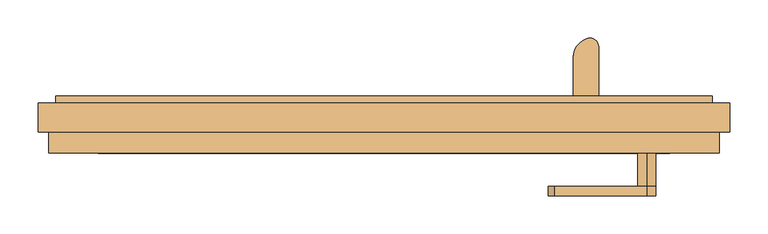
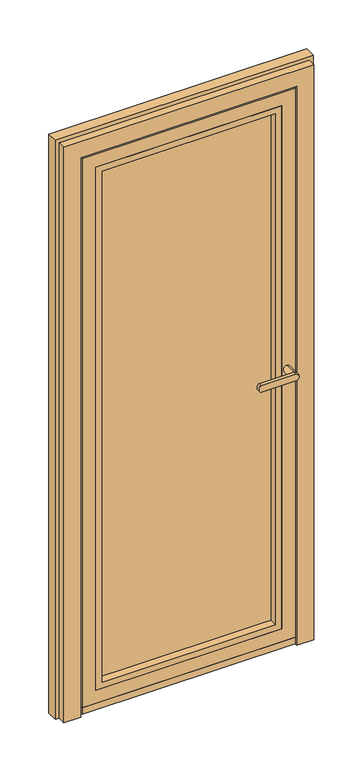
"""IFC4 building model written with IfcOpenShell, lengths in millimetres: door geometry, Schueco_FWS_ADS-75-HD-HI_out_Family-01 : FWS SI insert unit."""

from ifc_helpers import new_model, si_unit, point, frame, frame_2d, origin, place, context, project, spatial, polyline, circle_curve, ellipse_curve, trimmed, segment, composite_curve, outline, extrude, faceted_brep, source, transform, mapped, element, save
from ifc_brep_helpers import plane_surface, cylinder_surface, extruded_surface, advanced_brep


def door_b175160b(model_context):
    return source(origin(), model_context, "Body", "SolidModel", [
        extrude(outline(composite_curve([segment(polyline([(248.3337564, 8.9997177), (248.3337564, 59.1618682)]), True, "CONTINUOUS"), segment(trimmed(circle_curve(frame_2d((275.512174, 59.1618682)), 27.1784177), [point((248.3337564, 59.1618682))], [point((265.9750784, 84.6120194))], False, "CARTESIAN"), True, "CONTINUOUS"), segment(trimmed(circle_curve(frame_2d((270.0525794, 73.7310321)), 11.6198924), [point((265.9750784, 84.6120194))], [point((281.6724718, 73.7310321))], False, "CARTESIAN"), True, "CONTINUOUS"), segment(polyline([(281.6724718, 73.7310321), (281.6724718, 8.9997177), (248.3337564, 8.9997177)]), True, "CONTINUOUS")], self_intersect=False)), frame((0.0, 0.0, 2053.9218203), z_axis=(0.0, 0.0, 1.0), x_axis=(1.0, 0.0, 0.0)), (0.0, 0.0, 1.0), 4.0),
        extrude(outline(polyline([(248.3337564, 12.9997177), (281.6724718, 12.9997177), (281.6724718, 8.9997177), (248.3337564, 8.9997177), (248.3337564, 12.9997177)])), frame((0.0, 0.0, 2023.9218203), z_axis=(0.0, 0.0, 1.0), x_axis=(1.0, 0.0, 0.0)), (0.0, 0.0, 1.0), 30.0),
        extrude(outline(polyline([(248.3337564, 12.9997177), (281.6724718, 12.9997177), (281.6724718, 8.9997177), (248.3337564, 8.9997177), (248.3337564, 12.9997177)])), frame((0.0, 0.0, 49.9218203), z_axis=(0.0, 0.0, 1.0), x_axis=(1.0, 0.0, 0.0)), (0.0, 0.0, 1.0), 30.0),
        extrude(outline(composite_curve([segment(polyline([(248.3337564, 8.9997177), (248.3337564, 59.1618682)]), True, "CONTINUOUS"), segment(trimmed(circle_curve(frame_2d((275.512174, 59.1618682)), 27.1784177), [point((248.3337564, 59.1618682))], [point((265.9750784, 84.6120194))], False, "CARTESIAN"), True, "CONTINUOUS"), segment(trimmed(circle_curve(frame_2d((270.0525794, 73.7310321)), 11.6198924), [point((265.9750784, 84.6120194))], [point((281.6724718, 73.7310321))], False, "CARTESIAN"), True, "CONTINUOUS"), segment(polyline([(281.6724718, 73.7310321), (281.6724718, 8.9997177), (248.3337564, 8.9997177)]), True, "CONTINUOUS")], self_intersect=False)), frame((0.0, 0.0, 45.9218203), z_axis=(0.0, 0.0, 1.0), x_axis=(1.0, 0.0, 0.0)), (0.0, 0.0, 1.0), 4.0),
        advanced_brep(
        [(277.718156, 57.5977179, 2053.9218203), (252.2840039, 72.2821425, 2053.9218203), (277.718156, 57.5977179, 49.9218203), (252.2840039, 72.2821425, 49.9218203)],
        [
            (0, 1, ellipse_curve(frame((265.0010799, 64.9399302, 2053.9218203), z_axis=(0.0, 0.0, 1.0000000000000002), x_axis=(0.5000002582658958, 0.866025254674503, 0.0)), 21.5840887, 14.6844171)),
            (1, 0, ellipse_curve(frame((265.0010799, 64.9399302, 2053.9218203), z_axis=(0.0, 0.0, 1.0000000000000002), x_axis=(0.5000002582658958, 0.866025254674503, 0.0)), 21.5840887, 14.6844171)),
            (2, 3, ellipse_curve(frame((265.0010799, 64.9399302, 49.9218203), z_axis=(0.0, 0.0, -1.0000000000000002), x_axis=(-0.866025254674503, 0.5000002582658958, 0.0)), 14.6844171, 21.5840887)),
            (3, 2, ellipse_curve(frame((265.0010799, 64.9399302, 49.9218203), z_axis=(0.0, 0.0, -1.0000000000000002), x_axis=(-0.866025254674503, 0.5000002582658958, 0.0)), 14.6844171, 21.5840887)),
            (0, 2),
            (3, 1),
        ],
        [
            plane_surface(frame((252.2840039, 72.2821425, 2053.9218203), z_axis=(0.0, 0.0, 1.0000000000000002), x_axis=(0.5000002582658958, 0.866025254674503, 0.0))),
            plane_surface(frame((252.2840039, 72.2821425, 49.9218203), z_axis=(0.0, 0.0, -1.0000000000000002), x_axis=(-0.5000002582658958, -0.866025254674503, 0.0))),
            extruded_surface(trimmed(ellipse_curve(frame((265.0010799, 64.9399302, 49.9218203), z_axis=(0.0, 0.0, -1.0000000000000002), x_axis=(-0.866025254674503, 0.5000002582658958, 0.0)), 14.6844171, 21.5840887), [point((252.2840039, 72.2821425, 49.9218203))], [point((277.718156, 57.5977179, 49.9218203))], True, "CARTESIAN"), (0.0, 0.0, -2004.0), 2004.0),
            extruded_surface(trimmed(ellipse_curve(frame((265.0010799, 64.9399302, 49.9218203), z_axis=(0.0, 0.0, -1.0000000000000002), x_axis=(-0.866025254674503, 0.5000002582658958, 0.0)), 14.6844171, 21.5840887), [point((277.718156, 57.5977179, 49.9218203))], [point((252.2840039, 72.2821425, 49.9218203))], True, "CARTESIAN"), (0.0, 0.0, -2004.0), 2004.0),
        ],
        [
            (0, [[1, 2]]),
            (1, [[3, 4]]),
            (2, [[5, -4, 6, -1]]),
            (3, [[-6, -3, -5, -2]]),
        ],
    ),
        advanced_brep(
        [(345.0010799, -122.0002518, 1030.9991882), (345.0010799, -122.0002518, 1054.9764498), (223.3392873, -122.0002518, 1054.9764498), (223.3392873, -122.0002518, 1030.9991882), (345.0010799, -109.5001648, 1054.9764498), (345.0010799, -109.5001648, 1030.9991882), (223.3392873, -109.5001648, 1030.9991882), (223.3392873, -109.5001648, 1054.9764498), (345.0010799, -66.0002823, 1030.9991882), (345.0010799, -66.0002823, 1054.9764498)],
        [
            (0, 1, circle_curve(frame((345.0010799, -122.0002518, 1042.987819), z_axis=(0.0, -1.0, 0.0), x_axis=(0.0, 0.0, 1.0)), 11.9886308)),
            (1, 2),
            (2, 3, ellipse_curve(frame((223.3392873, -122.0002518, 1042.987819), z_axis=(0.0, -1.0, 0.0), x_axis=(0.0, 0.0, -1.0)), 11.9886308, 7.9050795)),
            (3, 0),
            (4, 5, circle_curve(frame((345.0010799, -109.5001648, 1042.987819), z_axis=(0.0, -1.0, 0.0), x_axis=(0.0, 0.0, 1.0)), 11.9886308)),
            (5, 6),
            (6, 7, ellipse_curve(frame((223.3392873, -109.5001648, 1042.987819), z_axis=(0.0, 1.0, 0.0), x_axis=(0.0, 0.0, -1.0)), 11.9886308, 7.9050795)),
            (7, 4),
            (3, 6),
            (5, 0),
            (2, 7),
            (1, 4),
            (5, 4, circle_curve(frame((345.0010799, -109.5001648, 1042.987819), z_axis=(0.0, -1.0, 0.0), x_axis=(0.0, 0.0, 1.0)), 11.9886308)),
            (8, 9, circle_curve(frame((345.0010799, -66.0002823, 1042.987819), z_axis=(0.0, 1.0, 0.0), x_axis=(0.0, 0.0, 1.0)), 11.9886308)),
            (9, 8, circle_curve(frame((345.0010799, -66.0002823, 1042.987819), z_axis=(0.0, 1.0, 0.0), x_axis=(0.0, 0.0, 1.0)), 11.9886308)),
            (8, 5),
            (4, 9),
        ],
        [
            plane_surface(frame((223.3392873, -122.0002518, 1030.9991882), z_axis=(0.0, -1.0, 0.0), x_axis=(-1.0, 0.0, 0.0))),
            plane_surface(frame((223.3392873, -109.5001648, 1030.9991882), z_axis=(0.0, 1.0, 0.0), x_axis=(1.0, 0.0, 0.0))),
            plane_surface(frame((345.0010799, -122.0002518, 1030.9991882), z_axis=(0.0, 0.0, -1.0), x_axis=(0.0, 1.0, 0.0))),
            extruded_surface(trimmed(ellipse_curve(frame((223.3392873, -109.5001648, 1042.987819), z_axis=(0.0, 1.0, 0.0), x_axis=(0.0, 0.0, -1.0)), 11.9886308, 7.9050795), [point((223.3392873, -109.5001648, 1030.9991882))], [point((223.3392873, -109.5001648, 1054.9764498))], True, "CARTESIAN"), (0.0, 12.500086999999994, 0.0), 12.500086999999994),
            plane_surface(frame((223.3392873, -122.0002518, 1054.9764498), z_axis=(0.0, 0.0, 1.0), x_axis=(0.0, 1.0, 0.0))),
            cylinder_surface(frame((345.0010799, -109.5001648, 1042.987819), z_axis=(0.0, -1.0, 0.0), x_axis=(0.0, 0.0, 1.0)), 11.9886308),
            plane_surface(frame((345.0010799, -66.0002823, 1054.9764498), z_axis=(0.0, 1.0, 0.0), x_axis=(-1.0, 0.0, 0.0))),
            cylinder_surface(frame((345.0010799, -66.0002823, 1042.987819), z_axis=(0.0, -1.0, 0.0), x_axis=(0.0, 0.0, 1.0)), 11.9886308),
        ],
        [
            (0, [[1, 2, 3, 4]]),
            (1, [[5, 6, 7, 8]]),
            (2, [[9, -6, 10, -4]]),
            (3, [[11, -7, -9, -3]]),
            (4, [[12, -8, -11, -2]]),
            (5, [[-10, 13, -12, -1]]),
            (6, [[14, 15]]),
            (7, [[16, -5, 17, -14]]),
            (7, [[-17, -13, -16, -15]]),
        ],
    ),
        extrude(outline(polyline([(80.9218203, 327.0670787), (2027.0538178, 327.0670787), (2027.0538178, -327.0649188), (80.9218203, -327.0649188), (80.9218203, 327.0670787)]), holes=[polyline([(102.9234681, -305.063271), (2005.05217, -305.063271), (2005.05217, 305.0654309), (102.9234681, 305.0654309), (102.9234681, -305.063271)])]), frame((0.0, -66.0002823, 0.0), z_axis=(0.0, 1.0, 0.0), x_axis=(0.0, 0.0, 1.0)), (0.0, 0.0, 1.0), 28.0002823),
        faceted_brep([(-375.0649188, -66.0002823, 2075.0538178), (-375.0649188, -57.5000065, 2075.0538178), (-375.0649188, -57.5000065, 32.9218203), (-375.0649188, -66.0002823, 32.9218203), (375.0670787, -57.5000065, 32.9218203), (375.0670787, -66.0002823, 32.9218203), (385.0670787, -57.5000065, 22.9218203), (385.0670787, -57.5000065, 2085.0538178), (-385.0649188, -57.5000065, 2085.0538178), (-385.0649188, -57.5000065, 22.9218203), (375.0670787, -57.5000065, 2075.0538178), (375.0670787, -66.0002823, 2075.0538178), (-327.0649188, -66.0002823, 80.9218203), (-327.0649188, -66.0002823, 2027.0538178), (327.0670787, -66.0002823, 2027.0538178), (327.0670787, -66.0002823, 80.9218203), (-327.0649188, 0.0, 2027.0538178), (-327.0649188, 0.0, 80.9218203), (327.0670787, 0.0, 80.9218203), (327.0670787, 0.0, 2027.0538178), (-302.0649188, 0.0, 105.9218203), (-302.0649188, 0.0, 2002.0538178), (302.0670787, 0.0, 2002.0538178), (302.0670787, 0.0, 105.9218203), (-302.0649188, 8.9997177, 2002.0538178), (-302.0649188, 8.9997177, 105.9218203), (302.0670787, 8.9997177, 105.9218203), (302.0670787, 8.9997177, 2002.0538178), (-400.0649188, 8.9997177, 7.9218203), (-400.0649188, 8.9997177, 2100.0538178), (400.0670787, 8.9997177, 2100.0538178), (400.0670787, 8.9997177, 7.9218203), (-400.0649188, 0.4997603, 2100.0538178), (-400.0649188, 0.4997603, 7.9218203), (400.0670787, 0.4997603, 7.9218203), (400.0670787, 0.4997603, 2100.0538178), (-385.0649188, 0.4997603, 22.9218203), (-385.0649188, 0.4997603, 2085.0538178), (385.0670787, 0.4997603, 2085.0538178), (385.0670787, 0.4997603, 22.9218203)], [[[0, 1, 2, 3]], [[3, 2, 4, 5]], [[6, 7, 8, 9], [2, 1, 10, 4]], [[5, 4, 10, 11]], [[5, 11, 0, 3], [12, 13, 14, 15]], [[16, 13, 12, 17]], [[17, 12, 15, 18]], [[18, 15, 14, 19]], [[18, 19, 16, 17], [20, 21, 22, 23]], [[24, 21, 20, 25]], [[25, 20, 23, 26]], [[26, 23, 22, 27]], [[28, 29, 30, 31], [26, 27, 24, 25]], [[32, 29, 28, 33]], [[33, 28, 31, 34]], [[34, 31, 30, 35]], [[34, 35, 32, 33], [36, 37, 38, 39]], [[8, 37, 36, 9]], [[9, 36, 39, 6]], [[6, 39, 38, 7]], [[11, 10, 1, 0]], [[19, 14, 13, 16]], [[27, 22, 21, 24]], [[35, 30, 29, 32]], [[7, 38, 37, 8]]]),
        extrude(outline(polyline([(327.0670787, -38.0), (-327.0649188, -38.0), (-327.0649188, 0.0), (327.0670787, 0.0), (327.0670787, -38.0)])), frame((0.0, 0.0, 80.9218203), z_axis=(0.0, 0.0, 1.0), x_axis=(1.0, 0.0, 0.0)), (0.0, 0.0, 1.0), 1946.1319975),
        extrude(outline(composite_curve([segment(polyline([(-31.4439202, 22.9218203), (-31.4439202, 4.2174554)]), True, "CONTINUOUS"), segment(trimmed(circle_curve(frame_2d((-42.0962864, 17.038728)), 16.6690713), [point((-31.4439202, 4.2174554))], [point((-52.7486527, 4.2174554))], False, "CARTESIAN"), True, "CONTINUOUS"), segment(polyline([(-52.7486527, 4.2174554), (-52.7486527, 22.9218203), (-31.4439202, 22.9218203)]), True, "CONTINUOUS")], self_intersect=False)), frame((-375.0649188, 0.0, 0.0), z_axis=(1.0, 0.0, 0.0), x_axis=(0.0, 1.0, 0.0)), (0.0, 0.0, 1.0), 750.1319975),
        extrude(outline(polyline([(-375.0649188, -66.0002823), (-375.0649188, -57.5000065), (375.0670787, -57.5000065), (375.0670787, -66.0002823), (-375.0649188, -66.0002823)])), frame((0.0, 0.0, 7.9218203), z_axis=(0.0, 0.0, 1.0), x_axis=(1.0, 0.0, 0.0)), (0.0, 0.0, 1.0), 25.0),
        faceted_brep([(430.999943, 8.9997177, 2130.999943), (430.999943, 0.0, 2130.999943), (430.999943, 0.0, 0.0), (430.999943, 8.9997177, 0.0), (-454.0, 0.0, 0.0), (-454.0, 0.0, 2154.0), (454.0, 0.0, 2154.0), (454.0, 0.0, 0.0), (-430.999943, 0.0, 2130.999943), (-430.999943, 0.0, 0.0), (454.0, -38.0, 0.0), (440.0, -38.0, 0.0), (440.0, -66.0002823, 0.0), (380.0652914, -66.0002823, 0.0), (380.0652914, -57.5000065, 0.0), (394.9999487, -57.5000065, 0.0), (394.9999487, 0.4997603, 0.0), (404.9999827, 0.4997603, 0.0), (404.9999827, 8.9997177, 0.0), (-404.9999827, 8.9997177, 0.0), (-430.999943, 8.9997177, 0.0), (-430.999943, 8.9997177, 2130.999943), (404.9999827, 8.9997177, 2104.9999827), (-404.9999827, 8.9997177, 2104.9999827), (380.0652914, -66.0002823, 2080.0652914), (380.0652914, -57.5000065, 2080.0652914), (-380.0652914, -57.5000065, 0.0), (-394.9999487, -57.5000065, 0.0), (-394.9999487, -57.5000065, 2094.9999487), (394.9999487, -57.5000065, 2094.9999487), (-380.0652914, -57.5000065, 2080.0652914), (-440.0, -66.0002823, 0.0), (-380.0652914, -66.0002823, 0.0), (-380.0652914, -66.0002823, 2080.0652914), (440.0, -66.0002823, 2140.0), (-440.0, -66.0002823, 2140.0), (440.0, -38.0, 2140.0), (-454.0, -38.0, 0.0), (-440.0, -38.0, 0.0), (-440.0, -38.0, 2140.0), (454.0, -38.0, 2154.0), (-454.0, -38.0, 2154.0), (-404.9999827, 0.4997603, 0.0), (-394.9999487, 0.4997603, 0.0), (404.9999827, 0.4997603, 2104.9999827), (-404.9999827, 0.4997603, 2104.9999827), (394.9999487, 0.4997603, 2094.9999487), (-394.9999487, 0.4997603, 2094.9999487)], [[[0, 1, 2, 3]], [[4, 5, 6, 7, 2, 1, 8, 9]], [[3, 2, 7, 10, 11, 12, 13, 14, 15, 16, 17, 18]], [[19, 20, 21, 0, 3, 18, 22, 23]], [[24, 25, 14, 13]], [[26, 27, 28, 29, 15, 14, 25, 30]], [[31, 32, 33, 24, 13, 12, 34, 35]], [[34, 12, 11, 36]], [[37, 38, 39, 36, 11, 10, 40, 41]], [[4, 9, 20, 19, 42, 43, 27, 26, 32, 31, 38, 37]], [[20, 9, 8, 21]], [[18, 17, 44, 22]], [[42, 19, 23, 45]], [[32, 26, 30, 33]], [[31, 35, 39, 38]], [[4, 37, 41, 5]], [[6, 40, 10, 7]], [[43, 42, 45, 44, 17, 16, 46, 47]], [[16, 15, 29, 46]], [[27, 43, 47, 28]], [[21, 8, 1, 0]], [[33, 30, 25, 24]], [[35, 34, 36, 39]], [[23, 22, 44, 45]], [[5, 41, 40, 6]], [[47, 46, 29, 28]]]),
    ])


if __name__ == "__main__":
    model = new_model("IFC4")
    model_context = context("Model", 3, world=origin())
    ifc_project = project(units=[si_unit("LENGTHUNIT", "METRE", prefix="MILLI")], contexts=[model_context])
    site = spatial("IfcSite", under=ifc_project)
    building = spatial("IfcBuilding", under=site)
    placement = place(None, origin())
    door_shape = door_b175160b(model_context)
    element("IfcDoor", 1, ObjectType="Schueco_FWS_ADS-75-HD-HI_out_Family-01 : FWS SI insert unit", at=placement, inside=building, context=model_context, shape_type="MappedRepresentation", body=[
        mapped(door_shape, transform((0.0, 0.0, 0.0), x_axis=(1.0, 0.0, 0.0), y_axis=(0.0, 1.0, 0.0), z_axis=(0.0, 0.0, 1.0))),
    ])
    save(model, "model.ifc")

# Revit data of these elements
# Type "Schueco_FWS_ADS-75-HD-HI_out_Family-01 : FWS SI insert unit"
#   Type Mark = "50"
#   __NOTE__ = "Data describes the optimum values of the entire system. The properites of a selected design option have to be determined on an individual basis!"
#   Wind load resistance = "Class 2"
#   Watertightness = "Class 5A"
#   Thermal insulation = "Uf = 1.4 W/(m²K)"
#   Sound insulation = "RW 43 db"
#   Schueco thermal insulation standard = "Highly thermally insulated"
#   Opening type = "Outward-opening, Flush-fitted"
#   Model = "Schueco ADS 75 HD.HI"
#   Mechanical loading = "Class 2"
#   Maximum leaf width in mm = "1400"
#   Maximum leaf weight in kg = "200"
#   Maximum leaf height in mm = "3000"
#   Material = "Aluminium"
#   Construction Type = "Door, single-leaf, outward-opening"
#   Manufacturer = "Schueco International KG"
#   Long term functionality = "Class 6"
#   Glazing data = "Triple glazing 38mm"
#   Façade insert unit = "yes"
#   Family creation date = "08.2017"
#   Description = "Schueco Aluminium Door System (ADS)"
#   Burglar resistance = "Class RC 3"
#   Areas of use = "Public buildings"
#   Analytic Construction = "<None>"
#   Air permeability = "Class 2"
#   Width [instance default] = 1464.636 mm
#   Leaf opening angle [instance default] = 0.00°
#   IOf_T = 38 mm
#   Height [instance default] = 2388.68 mm
#   Glazing area [instance default] = 2.47294 m²
#   Distance from bottom to handles [instance default] = 1050 mm
#   Clear opening width [instance default] = 1316.636 mm
#   Standard threshold = no
#   Low level threshold = yes
#   Handles = yes
#   FWS SI insert unit = yes
#   FWS HI insert unit = no
#   Glass = none
#   Frame = Alu
#   Fittings = none
# Element 1 (IfcDoor, "Schueco_FWS_ADS-75-HD-HI_out_Family-01 : FWS SI insert unit")
#   Width = 908 mm
#   Height = 2154 mm
#   Glazing area = 1.14518 m²
#   Clear opening width = 760 mm
#   Materials on its faces: "Alu", "Glass"
# Materials
#   "Alu": class "Glas", colour RGB 140 140 140, transparency 0
#   "Glass": class "Glass", colour RGB 128 128 255, transparency 0.75, Description = "Soda Lime Glass", Cost = 0
